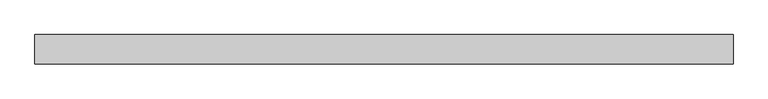
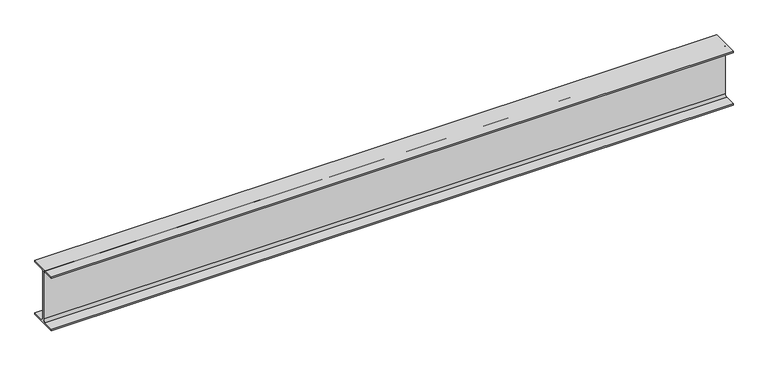
"""IFC4 building model written with IfcOpenShell, lengths in millimetres: beam geometry, 0912_Steel Framing_H-KSD3502 : H_SB_AR_S02_H-300x150x6.5x9_Stair."""

from ifc_helpers import new_model, si_unit, point, frame, frame_2d, origin, place, context, project, spatial, polyline, circle_curve, trimmed, segment, composite_curve, outline, extrude, source, transform, mapped, element, save


def beam_dad7a266(model_context):
    return source(origin(), model_context, "Body", "SweptSolid", [
        extrude(outline(composite_curve([segment(polyline([(75.0, -141.0), (75.0, -150.0), (-75.0, -150.0), (-75.0, -141.0), (-16.25, -141.0)]), True, "CONTINUOUS"), segment(trimmed(circle_curve(frame_2d((-16.25, -128.0)), 13.0), [point((-16.25, -141.0))], [point((-3.25, -128.0))], True, "CARTESIAN"), True, "CONTINUOUS"), segment(polyline([(-3.25, -128.0), (-3.25, 128.0)]), True, "CONTINUOUS"), segment(trimmed(circle_curve(frame_2d((-16.25, 128.0)), 13.0), [point((-3.25, 128.0))], [point((-16.25, 141.0))], True, "CARTESIAN"), True, "CONTINUOUS"), segment(polyline([(-16.25, 141.0), (-75.0, 141.0), (-75.0, 150.0), (75.0, 150.0), (75.0, 141.0), (16.25, 141.0)]), True, "CONTINUOUS"), segment(trimmed(circle_curve(frame_2d((16.25, 128.0)), 13.0), [point((16.25, 141.0))], [point((3.25, 128.0))], True, "CARTESIAN"), True, "CONTINUOUS"), segment(polyline([(3.25, 128.0), (3.25, -128.0)]), True, "CONTINUOUS"), segment(trimmed(circle_curve(frame_2d((16.25, -128.0)), 13.0), [point((3.25, -128.0))], [point((16.25, -141.0))], True, "CARTESIAN"), True, "CONTINUOUS"), segment(polyline([(16.25, -141.0), (75.0, -141.0)]), True, "CONTINUOUS")], self_intersect=False)), frame((-1787.3, 0.0, 0.0), z_axis=(1.0, 0.0, 0.0), x_axis=(0.0, 1.0, 0.0)), (0.0, 0.0, 1.0), 3574.6),
    ])


if __name__ == "__main__":
    model = new_model("IFC4")
    model_context = context("Model", 3, world=origin())
    ifc_project = project(units=[si_unit("LENGTHUNIT", "METRE", prefix="MILLI")], contexts=[model_context])
    site = spatial("IfcSite", under=ifc_project)
    building = spatial("IfcBuilding", under=site)
    placement = place(None, origin())
    beam_shape = beam_dad7a266(model_context)
    element("IfcBeam", 1, ObjectType="0912_Steel Framing_H-KSD3502 : H_SB_AR_S02_H-300x150x6.5x9_Stair", at=placement, inside=building, context=model_context, shape_type="MappedRepresentation", body=[
        mapped(beam_shape, transform((0.0, 0.0, 0.0), x_axis=(1.0, 0.0, 0.0), y_axis=(0.0, 1.0, 0.0), z_axis=(0.0, 0.0, 1.0))),
    ])
    save(model, "model.ifc")

# Revit data of these elements
# Type "0912_Steel Framing_H-KSD3502 : H_SB_AR_S02_H-300x150x6.5x9_Stair"
#   H_Q'ty Cal Type Tag = "SB-Q2"
#   H_WM Code_1 = "S01AA073-00001 |  | TON | Main Steel Structure Fabrication Work | Shelter/Building | Medium Steel - Standard |  |  |  |  |  |  | Material: (   ) | (90)KG/M>Weight≥(30)KG/M | S01AA073-00001 Main Steel Structure Fabrication Work Shelter/Building Medium Steel - Standard         | - Material: ( ASTM A36 )\n- (90)KG/M>Weight≥(30)KG/M"
#   H_WM Code_2 = "S03AA083-00001 |  | TON | Main Steel Structure Erection Work | Shelter/Building | Medium Steel |  |  |  |  |  |  | Material: (   ) | S03AA083-00001 Main Steel Structure Erection Work Shelter/Building Medium Steel         | - Material: ( ASTM A36 )"
#   H_WM Code_3 = "S01AA009-00001 |  | TON | Main Steel Structure Fabrication Work | Shelter/Building | Plates - Gusset, Stiffener, ETC | Material: (   ) | S01AA009-00001 Main Steel Structure Fabrication Work Shelter/Building Plates - Gusset, Stiffener, ETC         |"
#   H_WM Code_4 = "S41AA051-00001 |  | M2 | Steel Structure Paint Work | Shelter/Building | for Non-Fireproofed Steel Surface |  |  |  |  |  |  | Material: (   ) | S41AA051-00001 Steel Structure Paint Work Shelter/Building for Non-Fireproofed Steel Surface         |"
#   Width = 15.0 cm
#   Web Thickness = 0.65 cm
#   Web Fillet = 1.3 cm
#   Warping Constant = 107000.0 cm⁶
#   W = 0
#   Torsional Moment of Inertia = 9.9539 cm⁴
#   Section Area = 46.78 cm²
#   Plastic Modulus weak axis = 105.0 cm³
#   Plastic Modulus strong axis = 542.0 cm³
#   Perimeter = 1.17 m²/m
#   Nominal Weight = 36.70 kgf/m
#   Moment of Inertia weak axis = 508.00 cm⁴
#   Moment of Inertia strong axis = 7210.00 cm⁴
#   Height = 30.0 cm
#   Flange Thickness = 0.9 cm
#   Elastic Modulus weak axis = 67.7 cm³
#   Elastic Modulus strong axis = 481.0 cm³
#   Centroid Vertical = 15.0 cm
#   Centroid Horizontal = 7.5 cm
#   Ix = 72100000
#   Length [instance default] = 1524 mm
#   Zx = 542000
#   b = 150 mm
#   h = 300 mm
#   r = 13 mm
#   s = 6.5 mm
#   t = 9 mm
#   A = 0.004678 m²
#   Structural Material [instance default] = Steel, 45-345
#   Assembly Code = ""
# Element 1 (IfcBeam, "0912_Steel Framing_H-KSD3502 : H_SB_AR_S02_H-300x150x6.5x9_Stair")
#   Materials on its faces: "Steel, 45-345"
# Materials
#   "Steel, 45-345": class "Metal", colour RGB 189 187 185, transparency 0, Description = "Steel 345 MPa", Cost = 0
